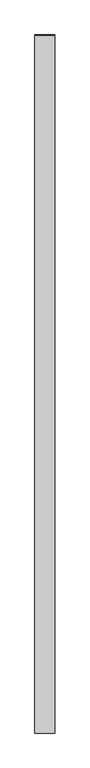
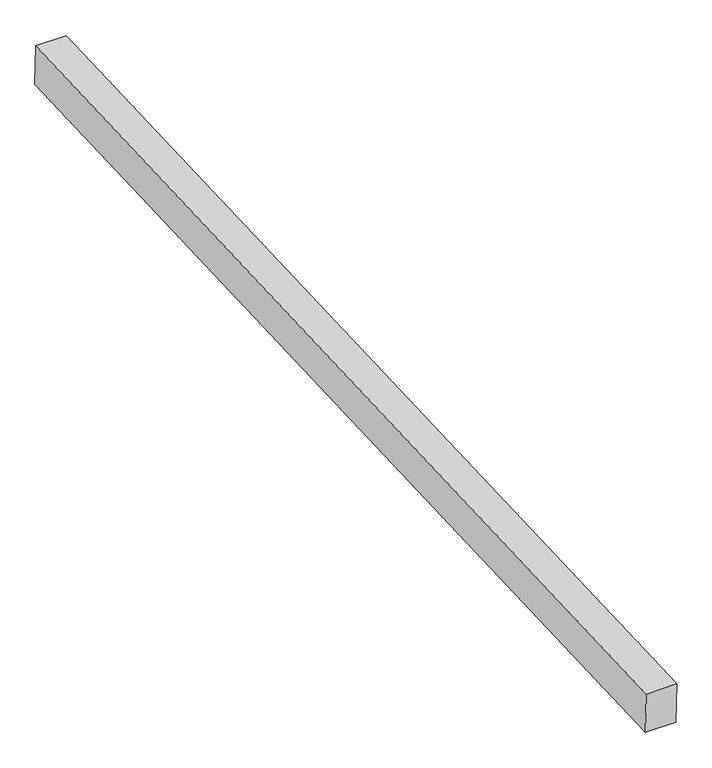
"""IFC4 building model written with IfcOpenShell, lengths in millimetres: proxy geometry, Generic Models 7:Generic Models 1:8:Generic Models 1:8 : Generic Models 7:Generic Models 1:337419:37 : Generic Models 7:Generic Models 1:8:Generic Models 1:8 : Generic Models 7:Generic Models 1:337419:315935."""

from ifc_helpers import new_model, si_unit, frame, origin, place, context, project, spatial, polyline, outline, extrude, source, transform, mapped, element, save


def generic_models_a6d960e6(model_context):
    return source(origin(), model_context, "Body", "SweptSolid", [
        extrude(outline(polyline([(-581229.2495411, 3818.908703), (-576356.3266468, 4021.9471569), (-576348.7597251, 3831.5971524), (-581221.3189223, 3628.5738526), (-581229.2495411, 3818.908703)])), frame((665972.5117239, 0.0, 0.0), z_axis=(1.0, 0.0, 0.0), x_axis=(0.0, 1.0, 0.0)), (0.0, 0.0, 1.0), 139.7),
    ])


if __name__ == "__main__":
    model = new_model("IFC4")
    model_context = context("Model", 3, world=origin())
    ifc_project = project(units=[si_unit("LENGTHUNIT", "METRE", prefix="MILLI")], contexts=[model_context])
    site = spatial("IfcSite", under=ifc_project)
    building = spatial("IfcBuilding", under=site)
    placement = place(None, origin())
    generic_models_shape = generic_models_a6d960e6(model_context)
    element("IfcBuildingElementProxy", 1, Name="Generic Models 7:Generic Models 1:8:Generic Models 1:8 : Generic Models 7:Generic Models 1:337419:37 : Generic Models 7:Generic Models 1:8:Generic Models 1:8 : Generic Models 7:Generic Models 1:337419:315935", ObjectType="Generic Models 7:Generic Models 1:8:Generic Models 1:8 : Generic Models 7:Generic Models 1:337419:37 : Generic Models 7:Generic Models 1:8:Generic Models 1:8 : Generic Models 7:Generic Models 1:337419:315935", at=placement, inside=building, context=model_context, shape_type="MappedRepresentation", body=[
        mapped(generic_models_shape, transform((0.0, 0.0, 0.0), x_axis=(1.0, 0.0, 0.0), y_axis=(0.0, 1.0, 0.0), z_axis=(0.0, 0.0, 1.0))),
    ])
    save(model, "model.ifc")

# Revit data of these elements
# Type "Generic Models 7:Generic Models 1:8:Generic Models 1:8 : Generic Models 7:Generic Models 1:337419:37 : Generic Models 7:Generic Models 1:8:Generic Models 1:8 : Generic Models 7:Generic Models 1:337419:315935"
#   NameOverride = "Generic Models 7:Generic Models 1:8:Generic Models 1:8 : Generic Models 7:Generic Models 1:337419:315935"
#   ObjectTypeOverride = "Generic Models 1:8 : Generic Models 7:Generic Models 1:337419"
#   Reference = "Generic Models 1"
#   Tag = "315935"
# Element 1 (IfcBuildingElementProxy, "Generic Models 7:Generic Models 1:8:Generic Models 1:8 : Generic Models 7:Generic Models 1:337419:37 : Generic Models 7:Generic Models 1:8:Generic Models 1:8 : Generic Models 7:Generic Models 1:337419:315935")
#   Materials on its faces: "5 1/2\" X 7 1/2\" EXTERIOR GRADE GLULAM BEAMS"
# Materials
#   "5 1/2\" X 7 1/2\" EXTERIOR GRADE GLULAM BEAMS": class "Wood", colour RGB 183 134 68, transparency 0, Keynote = "M06181300.01", Description = "Pinus Echinata", Cost = 0
